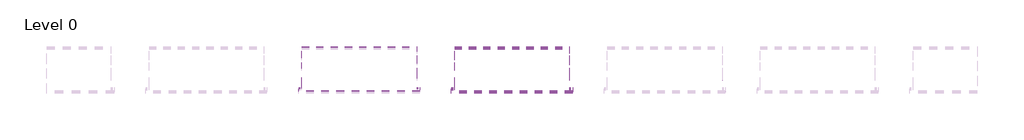
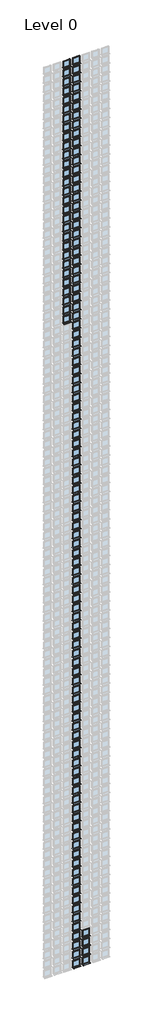
# One storey, part 12 of 75: 133 windows.
"""IFC4 building model written with IfcOpenShell, lengths in millimetres."""

import ifcopenshell
import ifcopenshell.guid

model = None  # the IFC model being written
_history = None  # IfcOwnerHistory: only IFC2X3 demands one
_inside = {}  # id of a spatial element -> (the spatial element, [elements in it])
_under = {}  # id of a project, library or spatial element -> (it, [spatial elements below it])
_declared = {}  # id of a project -> (the project, [libraries it declares])
_typed = {}  # id of a type object -> (the type object, [elements of that type])
_made_of = {}  # id of a material, layer set ... -> (it, [elements and type objects made of it])


def new_model(schema):
    """Start an empty IFC model of exactly this schema.

    Asked for "IFC4X3", IfcOpenShell would pick the latest addendum, in which some entities
    have other attributes; the version numbers below select the first issue.
    IFC2X3 requires an IfcOwnerHistory on every rooted entity: one is made here for all.
    """
    global model, _history
    if schema == "IFC4X3":
        model = ifcopenshell.file(schema_version=(4, 3, 0, 0))
    else:
        model = ifcopenshell.file(schema=schema)
    _inside.clear()
    _under.clear()
    _declared.clear()
    _typed.clear()
    _made_of.clear()
    _history = None
    if model.schema == "IFC2X3":
        org = make("IfcOrganization", Name="unknown")
        user = make(
            "IfcPersonAndOrganization",
            ThePerson=make("IfcPerson", FamilyName="unknown"),
            TheOrganization=org,
        )
        app = make(
            "IfcApplication",
            ApplicationDeveloper=org,
            Version="unknown",
            ApplicationFullName="unknown",
            ApplicationIdentifier="unknown",
        )
        _history = make(
            "IfcOwnerHistory",
            OwningUser=user,
            OwningApplication=app,
            ChangeAction="ADDED",
            CreationDate=0,
        )
    return model


def make(cls, **values):
    """One entity of the class cls with the attributes given. An attribute that is None is left unset."""
    return model.create_entity(
        cls, **{name: value for name, value in values.items() if value is not None}
    )


def rooted(cls, **values):
    """An entity with a GlobalId (a new one), such as an element, a storey or a relation."""
    return make(cls, GlobalId=ifcopenshell.guid.new(), OwnerHistory=_history, **values)


def si_unit(unit_type, name, prefix=None):
    """IfcSIUnit, for example si_unit("LENGTHUNIT", "METRE", prefix="MILLI")."""
    return make("IfcSIUnit", UnitType=unit_type, Prefix=prefix, Name=name)


def assignment(units):
    """IfcUnitAssignment: the units of a project."""
    return None if units is None else make("IfcUnitAssignment", Units=units)


def point(xyz):
    """IfcCartesianPoint."""
    return None if xyz is None else make("IfcCartesianPoint", Coordinates=xyz)


def direction(xyz):
    """IfcDirection."""
    return None if xyz is None else make("IfcDirection", DirectionRatios=xyz)


def frame(location, z_axis=None, x_axis=None):
    """IfcAxis2Placement3D, a coordinate frame: its origin and axes. An axis left out is left unset."""
    return make(
        "IfcAxis2Placement3D",
        Location=point(location),
        Axis=direction(z_axis),
        RefDirection=direction(x_axis),
    )


def origin():
    """The frame at (0, 0, 0) with its axes left unset."""
    return frame((0.0, 0.0, 0.0))


def place(relative_to, where):
    """IfcLocalPlacement: puts the frame where relative to a parent placement (None: the world)."""
    return make(
        "IfcLocalPlacement", PlacementRelTo=relative_to, RelativePlacement=where
    )


def context(
    kind, dimensions, precision=None, world=None, true_north=None, identifier=None
):
    """IfcGeometricRepresentationContext, for example the 3D "Model" context."""
    return make(
        "IfcGeometricRepresentationContext",
        ContextIdentifier=identifier,
        ContextType=kind,
        CoordinateSpaceDimension=dimensions,
        Precision=precision,
        WorldCoordinateSystem=world,
        TrueNorth=true_north,
    )


def project(units=None, contexts=None):
    """IfcProject with its units and contexts."""
    return rooted(
        "IfcProject",
        Name="project",
        RepresentationContexts=contexts,
        UnitsInContext=assignment(units),
    )


def spatial(cls, under=None, at=None, **own):
    """A site, building, storey or space (cls), placed at a placement, below another one or the project."""
    s = rooted(cls, ObjectPlacement=at, **own)
    if under is not None:
        _under.setdefault(under.id(), (under, []))[1].append(s)
    return s


def polyline(points):
    """IfcPolyline through the points."""
    return make("IfcPolyline", Points=[point(p) for p in points])


def outline(outer, holes=None, kind="AREA"):
    """IfcArbitraryClosedProfileDef: a profile drawn as a closed curve; with holes, ...WithVoids."""
    if holes is None:
        return make("IfcArbitraryClosedProfileDef", ProfileType=kind, OuterCurve=outer)
    return make(
        "IfcArbitraryProfileDefWithVoids",
        ProfileType=kind,
        OuterCurve=outer,
        InnerCurves=holes,
    )


def extrude(swept, where, along, depth):
    """IfcExtrudedAreaSolid: the profile swept, set in the frame where, extruded along a direction by depth."""
    return make(
        "IfcExtrudedAreaSolid",
        SweptArea=swept,
        Position=where,
        ExtrudedDirection=direction(along),
        Depth=depth,
    )


def faces_of(points, faces, orient=None, outer=None):
    """IfcFace entities. A face is a list of loops; a loop is a list of indices into points, from 0.

    orient and outer hold one flag for each loop. By default every Orientation is true, the
    first loop of a face is its IfcFaceOuterBound and the others are IfcFaceBound.
    """
    made = []
    for i, loops in enumerate(faces):
        bounds = []
        for j, loop in enumerate(loops):
            is_outer = j == 0 if outer is None else outer[i][j]
            bounds.append(
                make(
                    "IfcFaceOuterBound" if is_outer else "IfcFaceBound",
                    Bound=make("IfcPolyLoop", Polygon=[points[k] for k in loop]),
                    Orientation=True if orient is None else orient[i][j],
                )
            )
        made.append(make("IfcFace", Bounds=bounds))
    return made


def faceted_brep(points, faces, orient=None, outer=None, voids=None):
    """IfcFacetedBrep: a solid bounded by flat faces; with voids (closed shells), ...WithVoids."""
    shared = [point(p) for p in points]
    hull = make("IfcClosedShell", CfsFaces=faces_of(shared, faces, orient, outer))
    if voids is None:
        return make("IfcFacetedBrep", Outer=hull)
    return make(
        "IfcFacetedBrepWithVoids",
        Outer=hull,
        Voids=[
            make(cls, CfsFaces=faces_of(shared, fs, o, b)) for cls, fs, o, b in voids
        ],
    )


def shape(context_of_items, identifier, shape_type, items):
    """IfcShapeRepresentation: the items that make up one representation, for example the "Body"."""
    return make(
        "IfcShapeRepresentation",
        ContextOfItems=context_of_items,
        RepresentationIdentifier=identifier,
        RepresentationType=shape_type,
        Items=items,
    )


def source(mapping_origin, context_of_items, identifier, shape_type, items):
    """IfcRepresentationMap: a shape defined once, which mapped items show again and again."""
    return make(
        "IfcRepresentationMap",
        MappingOrigin=mapping_origin,
        MappedRepresentation=shape(context_of_items, identifier, shape_type, items),
    )


def transform(
    local_origin,
    x_axis=None,
    y_axis=None,
    z_axis=None,
    scale=None,
    scale2=None,
    scale3=None,
    uniform=True,
):
    """IfcCartesianTransformationOperator3D, or its non-uniform kind. x_axis, y_axis, z_axis: its Axis1, 2, 3."""
    if uniform:
        return make(
            "IfcCartesianTransformationOperator3D",
            Axis1=direction(x_axis),
            Axis2=direction(y_axis),
            LocalOrigin=point(local_origin),
            Scale=scale,
            Axis3=direction(z_axis),
        )
    return make(
        "IfcCartesianTransformationOperator3DnonUniform",
        Axis1=direction(x_axis),
        Axis2=direction(y_axis),
        LocalOrigin=point(local_origin),
        Scale=scale,
        Axis3=direction(z_axis),
        Scale2=scale2,
        Scale3=scale3,
    )


def mapped(mapping_source, mapping_target):
    """IfcMappedItem: shows the shape of a source again, moved by a transform."""
    return make(
        "IfcMappedItem", MappingSource=mapping_source, MappingTarget=mapping_target
    )


def made_of(thing, what):
    """Note that an element or type object is made of a material, layer set ...; save() writes the relation."""
    if what is not None:
        _made_of.setdefault(what.id(), (what, []))[1].append(thing)
    return thing


def element(
    cls,
    number,
    at=None,
    inside=None,
    cuts=None,
    type_object=None,
    material=None,
    context=None,
    identifier="Body",
    shape_type=None,
    held_by="IfcProductDefinitionShape",
    body=None,
    shapes=None,
    **own,
):
    """One element of the class cls, such as IfcWall. Its Tag is "e" and its number.

    at: its placement. inside: the storey or other place that contains it. cuts: it is an
    opening in that element (IfcRelVoidsElement). A single representation is given by context,
    identifier, shape_type and body (its items); several are given by shapes. held_by: the class
    of the entity that holds the representations. save() writes the other relations.
    """
    e = rooted(cls, Tag="e%d" % number, ObjectPlacement=at, **own)
    if body is not None:
        shapes = [shape(context, identifier, shape_type, body)]
    if shapes is not None:
        e.Representation = make(held_by, Representations=shapes)
    if inside is not None:
        _inside.setdefault(inside.id(), (inside, []))[1].append(e)
    if cuts is not None:
        rooted(
            "IfcRelVoidsElement", RelatingBuildingElement=cuts, RelatedOpeningElement=e
        )
    if type_object is not None:
        _typed.setdefault(type_object.id(), (type_object, []))[1].append(e)
    return made_of(e, material)


def aggregate(whole, parts):
    """IfcRelAggregates: a whole, such as a stair, and the parts it consists of."""
    return rooted("IfcRelAggregates", RelatingObject=whole, RelatedObjects=parts)


def save(model, path):
    """Write the relations noted so far, then the file.

    IfcRelAggregates (storeys below a building ...), IfcRelContainedInSpatialStructure (elements
    in a storey), IfcRelDefinesByType, IfcRelAssociatesMaterial and IfcRelDeclares: one each for
    every whole, place, type object, material and project.
    """
    for whole, parts in _under.values():
        aggregate(whole, parts)
    for where, things in _inside.values():
        rooted(
            "IfcRelContainedInSpatialStructure",
            RelatedElements=things,
            RelatingStructure=where,
        )
    for kind, things in _typed.values():
        rooted("IfcRelDefinesByType", RelatedObjects=things, RelatingType=kind)
    for what, things in _made_of.values():
        rooted("IfcRelAssociatesMaterial", RelatedObjects=things, RelatingMaterial=what)
    for by, libraries in _declared.values():
        rooted("IfcRelDeclares", RelatingContext=by, RelatedDefinitions=libraries)
    model.write(path)


def windows_sgl_plain_square_green_b9caa461(model_context):
    return source(origin(), model_context, "Body", "SolidModel", [
        extrude(outline(polyline([(-480.0, -161.5434322), (-480.0, -136.5434322), (-455.0, -136.5434322), (-455.0, 20.4565678), (455.0, 20.4565678), (455.0, -136.5434322), (480.0, -136.5434322), (480.0, -161.5434322), (-480.0, -161.5434322)])), frame((0.0, 0.0, 1200.0), z_axis=(0.0, 0.0, 1.0), x_axis=(1.0, 0.0, 0.0)), (0.0, 0.0, 1.0), 25.0),
        faceted_brep([(-455.0, 20.4565678, 1200.0), (455.0, 20.4565678, 1200.0), (455.0, 20.4565678, 2110.0), (-455.0, 20.4565678, 2110.0), (-395.0, 20.4565678, 2050.0), (395.0, 20.4565678, 2050.0), (395.0, 20.4565678, 1275.0), (-395.0, 20.4565678, 1275.0), (-455.0, 103.4565678, 2110.0), (-455.0, 103.4565678, 1251.0), (-455.0, 118.4565678, 1249.68767), (-455.0, 118.4565678, 1244.7449676), (-455.0, 190.9565678, 1233.8088847), (-455.0, 190.9565678, 1200.0), (455.0, 103.4565678, 2110.0), (455.0, 103.4565678, 1251.0), (-415.0, 103.4565678, 2070.0), (-415.0, 103.4565678, 1263.0), (415.0, 103.4565678, 1263.0), (415.0, 103.4565678, 2070.0), (-415.0, 38.4565678, 2070.0), (-415.0, 38.4565678, 1263.0), (415.0, 38.4565678, 2070.0), (415.0, 38.4565678, 1263.0), (-395.0, 38.4565678, 2050.0), (-395.0, 38.4565678, 1275.0), (395.0, 38.4565678, 1275.0), (395.0, 38.4565678, 2050.0), (455.0, 190.9565678, 1200.0), (455.0, 190.9565678, 1233.8088847), (455.0, 118.4565678, 1244.7449676), (455.0, 118.4565678, 1249.68767)], [[[0, 1, 2, 3], [4, 5, 6, 7]], [[0, 3, 8, 9, 10, 11, 12, 13]], [[9, 8, 14, 15], [16, 17, 18, 19]], [[17, 16, 20, 21]], [[20, 22, 23, 21], [24, 25, 26, 27]], [[24, 4, 7, 25]], [[3, 2, 14, 8]], [[16, 19, 22, 20]], [[5, 4, 24, 27]], [[15, 14, 2, 1, 28, 29, 30, 31]], [[19, 18, 23, 22]], [[5, 27, 26, 6]], [[28, 1, 0, 13]], [[29, 28, 13, 12]], [[30, 29, 12, 11]], [[31, 30, 11, 10]], [[15, 31, 10, 9]], [[21, 23, 18, 17]], [[7, 6, 26, 25]]]),
        extrude(outline(polyline([(385.0, 67.4565678), (-385.0, 67.4565678), (-385.0, 91.4565678), (385.0, 91.4565678), (385.0, 67.4565678)])), frame((0.0, 0.0, 1293.0), z_axis=(0.0, 0.0, 1.0), x_axis=(1.0, 0.0, 0.0)), (0.0, 0.0, 1.0), 747.0),
        faceted_brep([(-425.0, 103.4565678, 2080.0), (-425.0, 109.2300705, 2080.0), (-425.0, 109.2300705, 1253.0), (-425.0, 103.4565678, 1253.0), (-415.0, 38.4565678, 2070.0), (-415.0, 103.4565678, 2070.0), (-415.0, 103.4565678, 1263.0), (-415.0, 38.4565678, 1263.0), (-375.0, 52.9494677, 2030.0), (-385.1480377, 38.4565678, 2040.1480377), (-385.1480377, 38.4565678, 1292.8519623), (-375.0, 52.9494677, 1303.0), (-375.0, 67.4565678, 2030.0), (-375.0, 67.4565678, 1303.0), (-385.0, 91.4565678, 2040.0), (-385.0, 67.4565678, 2040.0), (-385.0, 67.4565678, 1293.0), (-385.0, 91.4565678, 1293.0), (-375.0, 109.2300705, 2030.0), (-375.0, 91.4565678, 2030.0), (-375.0, 91.4565678, 1303.0), (-375.0, 109.2300705, 1303.0), (-392.4457548, 115.0035732, 2047.4457548), (-392.4457548, 115.0035732, 1285.5542452), (-414.2153903, 115.0035732, 2069.2153903), (-414.2153903, 115.0035732, 1263.7846097), (425.0, 109.2300705, 1253.0), (425.0, 103.4565678, 1253.0), (415.0, 103.4565678, 1263.0), (415.0, 38.4565678, 1263.0), (385.1480377, 38.4565678, 1292.8519623), (375.0, 52.9494677, 1303.0), (375.0, 67.4565678, 1303.0), (385.0, 67.4565678, 1293.0), (385.0, 91.4565678, 1293.0), (375.0, 91.4565678, 1303.0), (375.0, 109.2300705, 1303.0), (392.4457548, 115.0035732, 1285.5542452), (414.2153903, 115.0035732, 1263.7846097), (425.0, 109.2300705, 2080.0), (425.0, 103.4565678, 2080.0), (415.0, 103.4565678, 2070.0), (415.0, 38.4565678, 2070.0), (385.1480377, 38.4565678, 2040.1480377), (375.0, 52.9494677, 2030.0), (375.0, 67.4565678, 2030.0), (385.0, 67.4565678, 2040.0), (385.0, 91.4565678, 2040.0), (375.0, 91.4565678, 2030.0), (375.0, 109.2300705, 2030.0), (392.4457548, 115.0035732, 2047.4457548), (414.2153903, 115.0035732, 2069.2153903)], [[[0, 1, 2, 3]], [[4, 5, 6, 7]], [[8, 9, 10, 11]], [[12, 8, 11, 13]], [[14, 15, 16, 17]], [[18, 19, 20, 21]], [[22, 18, 21, 23]], [[1, 24, 25, 2]], [[3, 2, 26, 27]], [[7, 6, 28, 29]], [[11, 10, 30, 31]], [[13, 11, 31, 32]], [[17, 16, 33, 34]], [[21, 20, 35, 36]], [[23, 21, 36, 37]], [[2, 25, 38, 26]], [[27, 26, 39, 40]], [[29, 28, 41, 42]], [[31, 30, 43, 44]], [[32, 31, 44, 45]], [[34, 33, 46, 47]], [[36, 35, 48, 49]], [[37, 36, 49, 50]], [[26, 38, 51, 39]], [[40, 39, 1, 0]], [[3, 27, 40, 0], [5, 41, 28, 6]], [[42, 41, 5, 4]], [[7, 29, 42, 4], [9, 43, 30, 10]], [[44, 43, 9, 8]], [[45, 44, 8, 12]], [[15, 46, 33, 16], [13, 32, 45, 12]], [[47, 46, 15, 14]], [[17, 34, 47, 14], [19, 48, 35, 20]], [[49, 48, 19, 18]], [[50, 49, 18, 22]], [[24, 51, 38, 25], [23, 37, 50, 22]], [[39, 51, 24, 1]]]),
    ])


model = new_model("IFC4")

# Units and contexts
model_context = context("Model", 3, world=origin())
ifc_project = project(units=[si_unit("LENGTHUNIT", "METRE", prefix="MILLI")], contexts=[model_context])

# Site, building, storey
site = spatial("IfcSite", under=ifc_project)
building = spatial("IfcBuilding", under=site)
storey = spatial("IfcBuildingStorey", under=building, Name="Level 0", Elevation=0.0)

# Windows
placement = place(None, origin())
windows_sgl_plain_square_green_shape = windows_sgl_plain_square_green_b9caa461(model_context)
element("IfcWindow", 1, ObjectType="Windows_Sgl_Plain : Square Green", at=placement, inside=storey, context=model_context, shape_type="MappedRepresentation", body=[
    mapped(windows_sgl_plain_square_green_shape, transform((-36933.7647367, 3061.0736592, 41224.2424242), x_axis=(1.0, 0.0, 0.0), y_axis=(0.0, 1.0, 0.0), z_axis=(0.0, 0.0, 1.0))),
])
element("IfcWindow", 2, ObjectType="Windows_Sgl_Plain : Square Green", at=placement, inside=storey, context=model_context, shape_type="MappedRepresentation", body=[
    mapped(windows_sgl_plain_square_green_shape, transform((-38145.8859488, 3061.0736592, 113951.5151515), x_axis=(1.0, 0.0, 0.0), y_axis=(0.0, 1.0, 0.0), z_axis=(0.0, 0.0, 1.0))),
])
element("IfcWindow", 3, ObjectType="Windows_Sgl_Plain : Square Green", at=placement, inside=storey, context=model_context, shape_type="MappedRepresentation", body=[
    mapped(windows_sgl_plain_square_green_shape, transform((-38145.8859488, 3061.0736592, 115163.6363636), x_axis=(1.0, 0.0, 0.0), y_axis=(0.0, 1.0, 0.0), z_axis=(0.0, 0.0, 1.0))),
])
element("IfcWindow", 4, ObjectType="Windows_Sgl_Plain : Square Normal", at=placement, inside=storey, context=model_context, shape_type="MappedRepresentation", body=[
    mapped(windows_sgl_plain_square_green_shape, transform((-38145.8859488, 3061.0736592, 41224.2424242), x_axis=(1.0, 0.0, 0.0), y_axis=(0.0, 1.0, 0.0), z_axis=(0.0, 0.0, 1.0))),
])
element("IfcWindow", 5, ObjectType="Windows_Sgl_Plain : Square Normal", at=placement, inside=storey, context=model_context, shape_type="MappedRepresentation", body=[
    mapped(windows_sgl_plain_square_green_shape, transform((-38145.8859488, 3061.0736592, 42436.3636364), x_axis=(1.0, 0.0, 0.0), y_axis=(0.0, 1.0, 0.0), z_axis=(0.0, 0.0, 1.0))),
])
element("IfcWindow", 6, ObjectType="Windows_Sgl_Plain : Square Normal", at=placement, inside=storey, context=model_context, shape_type="MappedRepresentation", body=[
    mapped(windows_sgl_plain_square_green_shape, transform((-36933.7647367, 3061.0736592, 42436.3636364), x_axis=(1.0, 0.0, 0.0), y_axis=(0.0, 1.0, 0.0), z_axis=(0.0, 0.0, 1.0))),
])
element("IfcWindow", 7, ObjectType="Windows_Sgl_Plain : Square Normal", at=placement, inside=storey, context=model_context, shape_type="MappedRepresentation", body=[
    mapped(windows_sgl_plain_square_green_shape, transform((-38145.8859488, 3061.0736592, 43648.4848485), x_axis=(1.0, 0.0, 0.0), y_axis=(0.0, 1.0, 0.0), z_axis=(0.0, 0.0, 1.0))),
])
element("IfcWindow", 8, ObjectType="Windows_Sgl_Plain : Square Normal", at=placement, inside=storey, context=model_context, shape_type="MappedRepresentation", body=[
    mapped(windows_sgl_plain_square_green_shape, transform((-38145.8859488, 3061.0736592, 44860.6060606), x_axis=(1.0, 0.0, 0.0), y_axis=(0.0, 1.0, 0.0), z_axis=(0.0, 0.0, 1.0))),
])
element("IfcWindow", 9, ObjectType="Windows_Sgl_Plain : Square Normal", at=placement, inside=storey, context=model_context, shape_type="MappedRepresentation", body=[
    mapped(windows_sgl_plain_square_green_shape, transform((-38145.8859488, 3061.0736592, 46072.7272727), x_axis=(1.0, 0.0, 0.0), y_axis=(0.0, 1.0, 0.0), z_axis=(0.0, 0.0, 1.0))),
])
element("IfcWindow", 10, ObjectType="Windows_Sgl_Plain : Square Normal", at=placement, inside=storey, context=model_context, shape_type="MappedRepresentation", body=[
    mapped(windows_sgl_plain_square_green_shape, transform((-38145.8859488, 3061.0736592, 47284.8484848), x_axis=(1.0, 0.0, 0.0), y_axis=(0.0, 1.0, 0.0), z_axis=(0.0, 0.0, 1.0))),
])
element("IfcWindow", 11, ObjectType="Windows_Sgl_Plain : Square Normal", at=placement, inside=storey, context=model_context, shape_type="MappedRepresentation", body=[
    mapped(windows_sgl_plain_square_green_shape, transform((-38145.8859488, 3061.0736592, 48496.969697), x_axis=(1.0, 0.0, 0.0), y_axis=(0.0, 1.0, 0.0), z_axis=(0.0, 0.0, 1.0))),
])
element("IfcWindow", 12, ObjectType="Windows_Sgl_Plain : Square Normal", at=placement, inside=storey, context=model_context, shape_type="MappedRepresentation", body=[
    mapped(windows_sgl_plain_square_green_shape, transform((-38145.8859488, 3061.0736592, 49709.0909091), x_axis=(1.0, 0.0, 0.0), y_axis=(0.0, 1.0, 0.0), z_axis=(0.0, 0.0, 1.0))),
])
element("IfcWindow", 13, ObjectType="Windows_Sgl_Plain : Square Normal", at=placement, inside=storey, context=model_context, shape_type="MappedRepresentation", body=[
    mapped(windows_sgl_plain_square_green_shape, transform((-38145.8859488, 3061.0736592, 50921.2121212), x_axis=(1.0, 0.0, 0.0), y_axis=(0.0, 1.0, 0.0), z_axis=(0.0, 0.0, 1.0))),
])
element("IfcWindow", 14, ObjectType="Windows_Sgl_Plain : Square Normal", at=placement, inside=storey, context=model_context, shape_type="MappedRepresentation", body=[
    mapped(windows_sgl_plain_square_green_shape, transform((-38145.8859488, 3061.0736592, 52133.3333333), x_axis=(1.0, 0.0, 0.0), y_axis=(0.0, 1.0, 0.0), z_axis=(0.0, 0.0, 1.0))),
])
element("IfcWindow", 15, ObjectType="Windows_Sgl_Plain : Square Normal", at=placement, inside=storey, context=model_context, shape_type="MappedRepresentation", body=[
    mapped(windows_sgl_plain_square_green_shape, transform((-38145.8859488, 3061.0736592, 53345.4545455), x_axis=(1.0, 0.0, 0.0), y_axis=(0.0, 1.0, 0.0), z_axis=(0.0, 0.0, 1.0))),
])
element("IfcWindow", 16, ObjectType="Windows_Sgl_Plain : Square Normal", at=placement, inside=storey, context=model_context, shape_type="MappedRepresentation", body=[
    mapped(windows_sgl_plain_square_green_shape, transform((-38145.8859488, 3061.0736592, 54557.5757576), x_axis=(1.0, 0.0, 0.0), y_axis=(0.0, 1.0, 0.0), z_axis=(0.0, 0.0, 1.0))),
])
element("IfcWindow", 17, ObjectType="Windows_Sgl_Plain : Square Normal", at=placement, inside=storey, context=model_context, shape_type="MappedRepresentation", body=[
    mapped(windows_sgl_plain_square_green_shape, transform((-38145.8859488, 3061.0736592, 55769.6969697), x_axis=(1.0, 0.0, 0.0), y_axis=(0.0, 1.0, 0.0), z_axis=(0.0, 0.0, 1.0))),
])
element("IfcWindow", 18, ObjectType="Windows_Sgl_Plain : Square Normal", at=placement, inside=storey, context=model_context, shape_type="MappedRepresentation", body=[
    mapped(windows_sgl_plain_square_green_shape, transform((-38145.8859488, 3061.0736592, 56981.8181818), x_axis=(1.0, 0.0, 0.0), y_axis=(0.0, 1.0, 0.0), z_axis=(0.0, 0.0, 1.0))),
])
element("IfcWindow", 19, ObjectType="Windows_Sgl_Plain : Square Normal", at=placement, inside=storey, context=model_context, shape_type="MappedRepresentation", body=[
    mapped(windows_sgl_plain_square_green_shape, transform((-38145.8859488, 3061.0736592, 58193.9393939), x_axis=(1.0, 0.0, 0.0), y_axis=(0.0, 1.0, 0.0), z_axis=(0.0, 0.0, 1.0))),
])
element("IfcWindow", 20, ObjectType="Windows_Sgl_Plain : Square Normal", at=placement, inside=storey, context=model_context, shape_type="MappedRepresentation", body=[
    mapped(windows_sgl_plain_square_green_shape, transform((-38145.8859488, 3061.0736592, 59406.0606061), x_axis=(1.0, 0.0, 0.0), y_axis=(0.0, 1.0, 0.0), z_axis=(0.0, 0.0, 1.0))),
])
element("IfcWindow", 21, ObjectType="Windows_Sgl_Plain : Square Normal", at=placement, inside=storey, context=model_context, shape_type="MappedRepresentation", body=[
    mapped(windows_sgl_plain_square_green_shape, transform((-38145.8859488, 3061.0736592, 60618.1818182), x_axis=(1.0, 0.0, 0.0), y_axis=(0.0, 1.0, 0.0), z_axis=(0.0, 0.0, 1.0))),
])
element("IfcWindow", 22, ObjectType="Windows_Sgl_Plain : Square Normal", at=placement, inside=storey, context=model_context, shape_type="MappedRepresentation", body=[
    mapped(windows_sgl_plain_square_green_shape, transform((-38145.8859488, 3061.0736592, 61830.3030303), x_axis=(1.0, 0.0, 0.0), y_axis=(0.0, 1.0, 0.0), z_axis=(0.0, 0.0, 1.0))),
])
element("IfcWindow", 23, ObjectType="Windows_Sgl_Plain : Square Normal", at=placement, inside=storey, context=model_context, shape_type="MappedRepresentation", body=[
    mapped(windows_sgl_plain_square_green_shape, transform((-38145.8859488, 3061.0736592, 63042.4242424), x_axis=(1.0, 0.0, 0.0), y_axis=(0.0, 1.0, 0.0), z_axis=(0.0, 0.0, 1.0))),
])
element("IfcWindow", 24, ObjectType="Windows_Sgl_Plain : Square Normal", at=placement, inside=storey, context=model_context, shape_type="MappedRepresentation", body=[
    mapped(windows_sgl_plain_square_green_shape, transform((-38145.8859488, 3061.0736592, 64254.5454545), x_axis=(1.0, 0.0, 0.0), y_axis=(0.0, 1.0, 0.0), z_axis=(0.0, 0.0, 1.0))),
])
element("IfcWindow", 25, ObjectType="Windows_Sgl_Plain : Square Normal", at=placement, inside=storey, context=model_context, shape_type="MappedRepresentation", body=[
    mapped(windows_sgl_plain_square_green_shape, transform((-38145.8859488, 3061.0736592, 65466.6666667), x_axis=(1.0, 0.0, 0.0), y_axis=(0.0, 1.0, 0.0), z_axis=(0.0, 0.0, 1.0))),
])
element("IfcWindow", 26, ObjectType="Windows_Sgl_Plain : Square Normal", at=placement, inside=storey, context=model_context, shape_type="MappedRepresentation", body=[
    mapped(windows_sgl_plain_square_green_shape, transform((-38145.8859488, 3061.0736592, 66678.7878788), x_axis=(1.0, 0.0, 0.0), y_axis=(0.0, 1.0, 0.0), z_axis=(0.0, 0.0, 1.0))),
])
element("IfcWindow", 27, ObjectType="Windows_Sgl_Plain : Square Normal", at=placement, inside=storey, context=model_context, shape_type="MappedRepresentation", body=[
    mapped(windows_sgl_plain_square_green_shape, transform((-38145.8859488, 3061.0736592, 67890.9090909), x_axis=(1.0, 0.0, 0.0), y_axis=(0.0, 1.0, 0.0), z_axis=(0.0, 0.0, 1.0))),
])
element("IfcWindow", 28, ObjectType="Windows_Sgl_Plain : Square Normal", at=placement, inside=storey, context=model_context, shape_type="MappedRepresentation", body=[
    mapped(windows_sgl_plain_square_green_shape, transform((-38145.8859488, 3061.0736592, 69103.030303), x_axis=(1.0, 0.0, 0.0), y_axis=(0.0, 1.0, 0.0), z_axis=(0.0, 0.0, 1.0))),
])
element("IfcWindow", 29, ObjectType="Windows_Sgl_Plain : Square Normal", at=placement, inside=storey, context=model_context, shape_type="MappedRepresentation", body=[
    mapped(windows_sgl_plain_square_green_shape, transform((-38145.8859488, 3061.0736592, 70315.1515152), x_axis=(1.0, 0.0, 0.0), y_axis=(0.0, 1.0, 0.0), z_axis=(0.0, 0.0, 1.0))),
])
element("IfcWindow", 30, ObjectType="Windows_Sgl_Plain : Square Normal", at=placement, inside=storey, context=model_context, shape_type="MappedRepresentation", body=[
    mapped(windows_sgl_plain_square_green_shape, transform((-38145.8859488, 3061.0736592, 71527.2727273), x_axis=(1.0, 0.0, 0.0), y_axis=(0.0, 1.0, 0.0), z_axis=(0.0, 0.0, 1.0))),
])
element("IfcWindow", 31, ObjectType="Windows_Sgl_Plain : Square Normal", at=placement, inside=storey, context=model_context, shape_type="MappedRepresentation", body=[
    mapped(windows_sgl_plain_square_green_shape, transform((-38145.8859488, 3061.0736592, 72739.3939394), x_axis=(1.0, 0.0, 0.0), y_axis=(0.0, 1.0, 0.0), z_axis=(0.0, 0.0, 1.0))),
])
element("IfcWindow", 32, ObjectType="Windows_Sgl_Plain : Square Normal", at=placement, inside=storey, context=model_context, shape_type="MappedRepresentation", body=[
    mapped(windows_sgl_plain_square_green_shape, transform((-38145.8859488, 3061.0736592, 73951.5151515), x_axis=(1.0, 0.0, 0.0), y_axis=(0.0, 1.0, 0.0), z_axis=(0.0, 0.0, 1.0))),
])
element("IfcWindow", 33, ObjectType="Windows_Sgl_Plain : Square Normal", at=placement, inside=storey, context=model_context, shape_type="MappedRepresentation", body=[
    mapped(windows_sgl_plain_square_green_shape, transform((-38145.8859488, 3061.0736592, 75163.6363636), x_axis=(1.0, 0.0, 0.0), y_axis=(0.0, 1.0, 0.0), z_axis=(0.0, 0.0, 1.0))),
])
element("IfcWindow", 34, ObjectType="Windows_Sgl_Plain : Square Normal", at=placement, inside=storey, context=model_context, shape_type="MappedRepresentation", body=[
    mapped(windows_sgl_plain_square_green_shape, transform((-38145.8859488, 3061.0736592, 76375.7575758), x_axis=(1.0, 0.0, 0.0), y_axis=(0.0, 1.0, 0.0), z_axis=(0.0, 0.0, 1.0))),
])
element("IfcWindow", 35, ObjectType="Windows_Sgl_Plain : Square Normal", at=placement, inside=storey, context=model_context, shape_type="MappedRepresentation", body=[
    mapped(windows_sgl_plain_square_green_shape, transform((-38145.8859488, 3061.0736592, 77587.8787879), x_axis=(1.0, 0.0, 0.0), y_axis=(0.0, 1.0, 0.0), z_axis=(0.0, 0.0, 1.0))),
])
element("IfcWindow", 36, ObjectType="Windows_Sgl_Plain : Square Normal", at=placement, inside=storey, context=model_context, shape_type="MappedRepresentation", body=[
    mapped(windows_sgl_plain_square_green_shape, transform((-38145.8859488, 3061.0736592, 78800.0), x_axis=(1.0, 0.0, 0.0), y_axis=(0.0, 1.0, 0.0), z_axis=(0.0, 0.0, 1.0))),
])
element("IfcWindow", 37, ObjectType="Windows_Sgl_Plain : Square Normal", at=placement, inside=storey, context=model_context, shape_type="MappedRepresentation", body=[
    mapped(windows_sgl_plain_square_green_shape, transform((-38145.8859488, 3061.0736592, 80012.1212121), x_axis=(1.0, 0.0, 0.0), y_axis=(0.0, 1.0, 0.0), z_axis=(0.0, 0.0, 1.0))),
])
element("IfcWindow", 38, ObjectType="Windows_Sgl_Plain : Square Normal", at=placement, inside=storey, context=model_context, shape_type="MappedRepresentation", body=[
    mapped(windows_sgl_plain_square_green_shape, transform((-38145.8859488, 3061.0736592, 81224.2424242), x_axis=(1.0, 0.0, 0.0), y_axis=(0.0, 1.0, 0.0), z_axis=(0.0, 0.0, 1.0))),
])
element("IfcWindow", 39, ObjectType="Windows_Sgl_Plain : Square Normal", at=placement, inside=storey, context=model_context, shape_type="MappedRepresentation", body=[
    mapped(windows_sgl_plain_square_green_shape, transform((-38145.8859488, 3061.0736592, 82436.3636364), x_axis=(1.0, 0.0, 0.0), y_axis=(0.0, 1.0, 0.0), z_axis=(0.0, 0.0, 1.0))),
])
element("IfcWindow", 40, ObjectType="Windows_Sgl_Plain : Square Normal", at=placement, inside=storey, context=model_context, shape_type="MappedRepresentation", body=[
    mapped(windows_sgl_plain_square_green_shape, transform((-38145.8859488, 3061.0736592, 83648.4848485), x_axis=(1.0, 0.0, 0.0), y_axis=(0.0, 1.0, 0.0), z_axis=(0.0, 0.0, 1.0))),
])
element("IfcWindow", 41, ObjectType="Windows_Sgl_Plain : Square Normal", at=placement, inside=storey, context=model_context, shape_type="MappedRepresentation", body=[
    mapped(windows_sgl_plain_square_green_shape, transform((-38145.8859488, 3061.0736592, 84860.6060606), x_axis=(1.0, 0.0, 0.0), y_axis=(0.0, 1.0, 0.0), z_axis=(0.0, 0.0, 1.0))),
])
element("IfcWindow", 42, ObjectType="Windows_Sgl_Plain : Square Normal", at=placement, inside=storey, context=model_context, shape_type="MappedRepresentation", body=[
    mapped(windows_sgl_plain_square_green_shape, transform((-38145.8859488, 3061.0736592, 86072.7272727), x_axis=(1.0, 0.0, 0.0), y_axis=(0.0, 1.0, 0.0), z_axis=(0.0, 0.0, 1.0))),
])
element("IfcWindow", 43, ObjectType="Windows_Sgl_Plain : Square Normal", at=placement, inside=storey, context=model_context, shape_type="MappedRepresentation", body=[
    mapped(windows_sgl_plain_square_green_shape, transform((-38145.8859488, 3061.0736592, 87284.8484848), x_axis=(1.0, 0.0, 0.0), y_axis=(0.0, 1.0, 0.0), z_axis=(0.0, 0.0, 1.0))),
])
element("IfcWindow", 44, ObjectType="Windows_Sgl_Plain : Square Normal", at=placement, inside=storey, context=model_context, shape_type="MappedRepresentation", body=[
    mapped(windows_sgl_plain_square_green_shape, transform((-38145.8859488, 3061.0736592, 88496.969697), x_axis=(1.0, 0.0, 0.0), y_axis=(0.0, 1.0, 0.0), z_axis=(0.0, 0.0, 1.0))),
])
element("IfcWindow", 45, ObjectType="Windows_Sgl_Plain : Square Normal", at=placement, inside=storey, context=model_context, shape_type="MappedRepresentation", body=[
    mapped(windows_sgl_plain_square_green_shape, transform((-38145.8859488, 3061.0736592, 89709.0909091), x_axis=(1.0, 0.0, 0.0), y_axis=(0.0, 1.0, 0.0), z_axis=(0.0, 0.0, 1.0))),
])
element("IfcWindow", 46, ObjectType="Windows_Sgl_Plain : Square Normal", at=placement, inside=storey, context=model_context, shape_type="MappedRepresentation", body=[
    mapped(windows_sgl_plain_square_green_shape, transform((-38145.8859488, 3061.0736592, 90921.2121212), x_axis=(1.0, 0.0, 0.0), y_axis=(0.0, 1.0, 0.0), z_axis=(0.0, 0.0, 1.0))),
])
element("IfcWindow", 47, ObjectType="Windows_Sgl_Plain : Square Normal", at=placement, inside=storey, context=model_context, shape_type="MappedRepresentation", body=[
    mapped(windows_sgl_plain_square_green_shape, transform((-38145.8859488, 3061.0736592, 96981.8181818), x_axis=(1.0, 0.0, 0.0), y_axis=(0.0, 1.0, 0.0), z_axis=(0.0, 0.0, 1.0))),
])
element("IfcWindow", 48, ObjectType="Windows_Sgl_Plain : Square Normal", at=placement, inside=storey, context=model_context, shape_type="MappedRepresentation", body=[
    mapped(windows_sgl_plain_square_green_shape, transform((-38145.8859488, 3061.0736592, 98193.9393939), x_axis=(1.0, 0.0, 0.0), y_axis=(0.0, 1.0, 0.0), z_axis=(0.0, 0.0, 1.0))),
])
element("IfcWindow", 49, ObjectType="Windows_Sgl_Plain : Square Normal", at=placement, inside=storey, context=model_context, shape_type="MappedRepresentation", body=[
    mapped(windows_sgl_plain_square_green_shape, transform((-38145.8859488, 3061.0736592, 99406.0606061), x_axis=(1.0, 0.0, 0.0), y_axis=(0.0, 1.0, 0.0), z_axis=(0.0, 0.0, 1.0))),
])
element("IfcWindow", 50, ObjectType="Windows_Sgl_Plain : Square Normal", at=placement, inside=storey, context=model_context, shape_type="MappedRepresentation", body=[
    mapped(windows_sgl_plain_square_green_shape, transform((-38145.8859488, 3061.0736592, 100618.1818182), x_axis=(1.0, 0.0, 0.0), y_axis=(0.0, 1.0, 0.0), z_axis=(0.0, 0.0, 1.0))),
])
element("IfcWindow", 51, ObjectType="Windows_Sgl_Plain : Square Normal", at=placement, inside=storey, context=model_context, shape_type="MappedRepresentation", body=[
    mapped(windows_sgl_plain_square_green_shape, transform((-38145.8859488, 3061.0736592, 101830.3030303), x_axis=(1.0, 0.0, 0.0), y_axis=(0.0, 1.0, 0.0), z_axis=(0.0, 0.0, 1.0))),
])
element("IfcWindow", 52, ObjectType="Windows_Sgl_Plain : Square Normal", at=placement, inside=storey, context=model_context, shape_type="MappedRepresentation", body=[
    mapped(windows_sgl_plain_square_green_shape, transform((-38145.8859488, 3061.0736592, 103042.4242424), x_axis=(1.0, 0.0, 0.0), y_axis=(0.0, 1.0, 0.0), z_axis=(0.0, 0.0, 1.0))),
])
element("IfcWindow", 53, ObjectType="Windows_Sgl_Plain : Square Normal", at=placement, inside=storey, context=model_context, shape_type="MappedRepresentation", body=[
    mapped(windows_sgl_plain_square_green_shape, transform((-38145.8859488, 3061.0736592, 104254.5454545), x_axis=(1.0, 0.0, 0.0), y_axis=(0.0, 1.0, 0.0), z_axis=(0.0, 0.0, 1.0))),
])
element("IfcWindow", 54, ObjectType="Windows_Sgl_Plain : Square Normal", at=placement, inside=storey, context=model_context, shape_type="MappedRepresentation", body=[
    mapped(windows_sgl_plain_square_green_shape, transform((-38145.8859488, 3061.0736592, 105466.6666667), x_axis=(1.0, 0.0, 0.0), y_axis=(0.0, 1.0, 0.0), z_axis=(0.0, 0.0, 1.0))),
])
element("IfcWindow", 55, ObjectType="Windows_Sgl_Plain : Square Normal", at=placement, inside=storey, context=model_context, shape_type="MappedRepresentation", body=[
    mapped(windows_sgl_plain_square_green_shape, transform((-38145.8859488, 3061.0736592, 106678.7878788), x_axis=(1.0, 0.0, 0.0), y_axis=(0.0, 1.0, 0.0), z_axis=(0.0, 0.0, 1.0))),
])
element("IfcWindow", 56, ObjectType="Windows_Sgl_Plain : Square Normal", at=placement, inside=storey, context=model_context, shape_type="MappedRepresentation", body=[
    mapped(windows_sgl_plain_square_green_shape, transform((-38145.8859488, 3061.0736592, 107890.9090909), x_axis=(1.0, 0.0, 0.0), y_axis=(0.0, 1.0, 0.0), z_axis=(0.0, 0.0, 1.0))),
])
element("IfcWindow", 57, ObjectType="Windows_Sgl_Plain : Square Normal", at=placement, inside=storey, context=model_context, shape_type="MappedRepresentation", body=[
    mapped(windows_sgl_plain_square_green_shape, transform((-38145.8859488, 3061.0736592, 109103.030303), x_axis=(1.0, 0.0, 0.0), y_axis=(0.0, 1.0, 0.0), z_axis=(0.0, 0.0, 1.0))),
])
element("IfcWindow", 58, ObjectType="Windows_Sgl_Plain : Square Normal", at=placement, inside=storey, context=model_context, shape_type="MappedRepresentation", body=[
    mapped(windows_sgl_plain_square_green_shape, transform((-38145.8859488, 3061.0736592, 110315.1515152), x_axis=(1.0, 0.0, 0.0), y_axis=(0.0, 1.0, 0.0), z_axis=(0.0, 0.0, 1.0))),
])
element("IfcWindow", 59, ObjectType="Windows_Sgl_Plain : Square Normal", at=placement, inside=storey, context=model_context, shape_type="MappedRepresentation", body=[
    mapped(windows_sgl_plain_square_green_shape, transform((-38145.8859488, 3061.0736592, 111527.2727273), x_axis=(1.0, 0.0, 0.0), y_axis=(0.0, 1.0, 0.0), z_axis=(0.0, 0.0, 1.0))),
])
element("IfcWindow", 60, ObjectType="Windows_Sgl_Plain : Square Normal", at=placement, inside=storey, context=model_context, shape_type="MappedRepresentation", body=[
    mapped(windows_sgl_plain_square_green_shape, transform((-38145.8859488, 3061.0736592, 112739.3939394), x_axis=(1.0, 0.0, 0.0), y_axis=(0.0, 1.0, 0.0), z_axis=(0.0, 0.0, 1.0))),
])
element("IfcWindow", 61, ObjectType="Windows_Sgl_Plain : Square Normal", at=placement, inside=storey, context=model_context, shape_type="MappedRepresentation", body=[
    mapped(windows_sgl_plain_square_green_shape, transform((-38145.8859488, 3061.0736592, 116375.7575758), x_axis=(1.0, 0.0, 0.0), y_axis=(0.0, 1.0, 0.0), z_axis=(0.0, 0.0, 1.0))),
])
element("IfcWindow", 62, ObjectType="Windows_Sgl_Plain : Square Normal", at=placement, inside=storey, context=model_context, shape_type="MappedRepresentation", body=[
    mapped(windows_sgl_plain_square_green_shape, transform((-38145.8859488, 3061.0736592, 117587.8787879), x_axis=(1.0, 0.0, 0.0), y_axis=(0.0, 1.0, 0.0), z_axis=(0.0, 0.0, 1.0))),
])
element("IfcWindow", 63, ObjectType="Windows_Sgl_Plain : Square Normal", at=placement, inside=storey, context=model_context, shape_type="MappedRepresentation", body=[
    mapped(windows_sgl_plain_square_green_shape, transform((-38145.8859488, 3061.0736592, 118800.0), x_axis=(1.0, 0.0, 0.0), y_axis=(0.0, 1.0, 0.0), z_axis=(0.0, 0.0, 1.0))),
])
element("IfcWindow", 64, ObjectType="Windows_Sgl_Plain : Square Normal", at=placement, inside=storey, context=model_context, shape_type="MappedRepresentation", body=[
    mapped(windows_sgl_plain_square_green_shape, transform((-38145.8859488, 3061.0736592, 120012.1212121), x_axis=(1.0, 0.0, 0.0), y_axis=(0.0, 1.0, 0.0), z_axis=(0.0, 0.0, 1.0))),
])
element("IfcWindow", 65, ObjectType="Windows_Sgl_Plain : Square Normal", at=placement, inside=storey, context=model_context, shape_type="MappedRepresentation", body=[
    mapped(windows_sgl_plain_square_green_shape, transform((-38145.8859488, 3061.0736592, 121224.2424242), x_axis=(1.0, 0.0, 0.0), y_axis=(0.0, 1.0, 0.0), z_axis=(0.0, 0.0, 1.0))),
])
element("IfcWindow", 66, ObjectType="Windows_Sgl_Plain : Square Normal", at=placement, inside=storey, context=model_context, shape_type="MappedRepresentation", body=[
    mapped(windows_sgl_plain_square_green_shape, transform((-38145.8859488, 3061.0736592, 122436.3636364), x_axis=(1.0, 0.0, 0.0), y_axis=(0.0, 1.0, 0.0), z_axis=(0.0, 0.0, 1.0))),
])
element("IfcWindow", 67, ObjectType="Windows_Sgl_Plain : Square Normal", at=placement, inside=storey, context=model_context, shape_type="MappedRepresentation", body=[
    mapped(windows_sgl_plain_square_green_shape, transform((-38145.8859488, 3061.0736592, 123648.4848485), x_axis=(1.0, 0.0, 0.0), y_axis=(0.0, 1.0, 0.0), z_axis=(0.0, 0.0, 1.0))),
])
element("IfcWindow", 68, ObjectType="Windows_Sgl_Plain : Square Normal", at=placement, inside=storey, context=model_context, shape_type="MappedRepresentation", body=[
    mapped(windows_sgl_plain_square_green_shape, transform((-39358.007161, 3061.0736592, 124860.6060606), x_axis=(1.0, 0.0, 0.0), y_axis=(0.0, 1.0, 0.0), z_axis=(0.0, 0.0, 1.0))),
])
element("IfcWindow", 69, ObjectType="Windows_Sgl_Plain : Square Normal", at=placement, inside=storey, context=model_context, shape_type="MappedRepresentation", body=[
    mapped(windows_sgl_plain_square_green_shape, transform((-38145.8859488, 3061.0736592, 124860.6060606), x_axis=(1.0, 0.0, 0.0), y_axis=(0.0, 1.0, 0.0), z_axis=(0.0, 0.0, 1.0))),
])
element("IfcWindow", 70, ObjectType="Windows_Sgl_Plain : Square Normal", at=placement, inside=storey, context=model_context, shape_type="MappedRepresentation", body=[
    mapped(windows_sgl_plain_square_green_shape, transform((-39358.007161, 3061.0736592, 126072.7272727), x_axis=(1.0, 0.0, 0.0), y_axis=(0.0, 1.0, 0.0), z_axis=(0.0, 0.0, 1.0))),
])
element("IfcWindow", 71, ObjectType="Windows_Sgl_Plain : Square Normal", at=placement, inside=storey, context=model_context, shape_type="MappedRepresentation", body=[
    mapped(windows_sgl_plain_square_green_shape, transform((-38145.8859488, 3061.0736592, 126072.7272727), x_axis=(1.0, 0.0, 0.0), y_axis=(0.0, 1.0, 0.0), z_axis=(0.0, 0.0, 1.0))),
])
element("IfcWindow", 72, ObjectType="Windows_Sgl_Plain : Square Normal", at=placement, inside=storey, context=model_context, shape_type="MappedRepresentation", body=[
    mapped(windows_sgl_plain_square_green_shape, transform((-39358.007161, 3061.0736592, 127284.8484848), x_axis=(1.0, 0.0, 0.0), y_axis=(0.0, 1.0, 0.0), z_axis=(0.0, 0.0, 1.0))),
])
element("IfcWindow", 73, ObjectType="Windows_Sgl_Plain : Square Normal", at=placement, inside=storey, context=model_context, shape_type="MappedRepresentation", body=[
    mapped(windows_sgl_plain_square_green_shape, transform((-38145.8859488, 3061.0736592, 127284.8484848), x_axis=(1.0, 0.0, 0.0), y_axis=(0.0, 1.0, 0.0), z_axis=(0.0, 0.0, 1.0))),
])
element("IfcWindow", 74, ObjectType="Windows_Sgl_Plain : Square Normal", at=placement, inside=storey, context=model_context, shape_type="MappedRepresentation", body=[
    mapped(windows_sgl_plain_square_green_shape, transform((-39358.007161, 3061.0736592, 128496.969697), x_axis=(1.0, 0.0, 0.0), y_axis=(0.0, 1.0, 0.0), z_axis=(0.0, 0.0, 1.0))),
])
element("IfcWindow", 75, ObjectType="Windows_Sgl_Plain : Square Normal", at=placement, inside=storey, context=model_context, shape_type="MappedRepresentation", body=[
    mapped(windows_sgl_plain_square_green_shape, transform((-38145.8859488, 3061.0736592, 128496.969697), x_axis=(1.0, 0.0, 0.0), y_axis=(0.0, 1.0, 0.0), z_axis=(0.0, 0.0, 1.0))),
])
element("IfcWindow", 76, ObjectType="Windows_Sgl_Plain : Square Normal", at=placement, inside=storey, context=model_context, shape_type="MappedRepresentation", body=[
    mapped(windows_sgl_plain_square_green_shape, transform((-39358.007161, 3061.0736592, 129709.0909091), x_axis=(1.0, 0.0, 0.0), y_axis=(0.0, 1.0, 0.0), z_axis=(0.0, 0.0, 1.0))),
])
element("IfcWindow", 77, ObjectType="Windows_Sgl_Plain : Square Normal", at=placement, inside=storey, context=model_context, shape_type="MappedRepresentation", body=[
    mapped(windows_sgl_plain_square_green_shape, transform((-38145.8859488, 3061.0736592, 129709.0909091), x_axis=(1.0, 0.0, 0.0), y_axis=(0.0, 1.0, 0.0), z_axis=(0.0, 0.0, 1.0))),
])
element("IfcWindow", 78, ObjectType="Windows_Sgl_Plain : Square Normal", at=placement, inside=storey, context=model_context, shape_type="MappedRepresentation", body=[
    mapped(windows_sgl_plain_square_green_shape, transform((-39358.007161, 3061.0736592, 130921.2121212), x_axis=(1.0, 0.0, 0.0), y_axis=(0.0, 1.0, 0.0), z_axis=(0.0, 0.0, 1.0))),
])
element("IfcWindow", 79, ObjectType="Windows_Sgl_Plain : Square Normal", at=placement, inside=storey, context=model_context, shape_type="MappedRepresentation", body=[
    mapped(windows_sgl_plain_square_green_shape, transform((-38145.8859488, 3061.0736592, 130921.2121212), x_axis=(1.0, 0.0, 0.0), y_axis=(0.0, 1.0, 0.0), z_axis=(0.0, 0.0, 1.0))),
])
element("IfcWindow", 80, ObjectType="Windows_Sgl_Plain : Square Normal", at=placement, inside=storey, context=model_context, shape_type="MappedRepresentation", body=[
    mapped(windows_sgl_plain_square_green_shape, transform((-39358.007161, 3061.0736592, 132133.3333333), x_axis=(1.0, 0.0, 0.0), y_axis=(0.0, 1.0, 0.0), z_axis=(0.0, 0.0, 1.0))),
])
element("IfcWindow", 81, ObjectType="Windows_Sgl_Plain : Square Normal", at=placement, inside=storey, context=model_context, shape_type="MappedRepresentation", body=[
    mapped(windows_sgl_plain_square_green_shape, transform((-38145.8859488, 3061.0736592, 132133.3333333), x_axis=(1.0, 0.0, 0.0), y_axis=(0.0, 1.0, 0.0), z_axis=(0.0, 0.0, 1.0))),
])
element("IfcWindow", 82, ObjectType="Windows_Sgl_Plain : Square Normal", at=placement, inside=storey, context=model_context, shape_type="MappedRepresentation", body=[
    mapped(windows_sgl_plain_square_green_shape, transform((-39358.007161, 3061.0736592, 133345.4545455), x_axis=(1.0, 0.0, 0.0), y_axis=(0.0, 1.0, 0.0), z_axis=(0.0, 0.0, 1.0))),
])
element("IfcWindow", 83, ObjectType="Windows_Sgl_Plain : Square Normal", at=placement, inside=storey, context=model_context, shape_type="MappedRepresentation", body=[
    mapped(windows_sgl_plain_square_green_shape, transform((-38145.8859488, 3061.0736592, 133345.4545455), x_axis=(1.0, 0.0, 0.0), y_axis=(0.0, 1.0, 0.0), z_axis=(0.0, 0.0, 1.0))),
])
element("IfcWindow", 84, ObjectType="Windows_Sgl_Plain : Square Normal", at=placement, inside=storey, context=model_context, shape_type="MappedRepresentation", body=[
    mapped(windows_sgl_plain_square_green_shape, transform((-39358.007161, 3061.0736592, 134557.5757576), x_axis=(1.0, 0.0, 0.0), y_axis=(0.0, 1.0, 0.0), z_axis=(0.0, 0.0, 1.0))),
])
element("IfcWindow", 85, ObjectType="Windows_Sgl_Plain : Square Normal", at=placement, inside=storey, context=model_context, shape_type="MappedRepresentation", body=[
    mapped(windows_sgl_plain_square_green_shape, transform((-38145.8859488, 3061.0736592, 134557.5757576), x_axis=(1.0, 0.0, 0.0), y_axis=(0.0, 1.0, 0.0), z_axis=(0.0, 0.0, 1.0))),
])
element("IfcWindow", 86, ObjectType="Windows_Sgl_Plain : Square Normal", at=placement, inside=storey, context=model_context, shape_type="MappedRepresentation", body=[
    mapped(windows_sgl_plain_square_green_shape, transform((-39358.007161, 3061.0736592, 135769.6969697), x_axis=(1.0, 0.0, 0.0), y_axis=(0.0, 1.0, 0.0), z_axis=(0.0, 0.0, 1.0))),
])
element("IfcWindow", 87, ObjectType="Windows_Sgl_Plain : Square Normal", at=placement, inside=storey, context=model_context, shape_type="MappedRepresentation", body=[
    mapped(windows_sgl_plain_square_green_shape, transform((-38145.8859488, 3061.0736592, 135769.6969697), x_axis=(1.0, 0.0, 0.0), y_axis=(0.0, 1.0, 0.0), z_axis=(0.0, 0.0, 1.0))),
])
element("IfcWindow", 88, ObjectType="Windows_Sgl_Plain : Square Normal", at=placement, inside=storey, context=model_context, shape_type="MappedRepresentation", body=[
    mapped(windows_sgl_plain_square_green_shape, transform((-39358.007161, 3061.0736592, 136981.8181818), x_axis=(1.0, 0.0, 0.0), y_axis=(0.0, 1.0, 0.0), z_axis=(0.0, 0.0, 1.0))),
])
element("IfcWindow", 89, ObjectType="Windows_Sgl_Plain : Square Normal", at=placement, inside=storey, context=model_context, shape_type="MappedRepresentation", body=[
    mapped(windows_sgl_plain_square_green_shape, transform((-38145.8859488, 3061.0736592, 136981.8181818), x_axis=(1.0, 0.0, 0.0), y_axis=(0.0, 1.0, 0.0), z_axis=(0.0, 0.0, 1.0))),
])
element("IfcWindow", 90, ObjectType="Windows_Sgl_Plain : Square Normal", at=placement, inside=storey, context=model_context, shape_type="MappedRepresentation", body=[
    mapped(windows_sgl_plain_square_green_shape, transform((-39358.007161, 3061.0736592, 138193.9393939), x_axis=(1.0, 0.0, 0.0), y_axis=(0.0, 1.0, 0.0), z_axis=(0.0, 0.0, 1.0))),
])
element("IfcWindow", 91, ObjectType="Windows_Sgl_Plain : Square Normal", at=placement, inside=storey, context=model_context, shape_type="MappedRepresentation", body=[
    mapped(windows_sgl_plain_square_green_shape, transform((-38145.8859488, 3061.0736592, 138193.9393939), x_axis=(1.0, 0.0, 0.0), y_axis=(0.0, 1.0, 0.0), z_axis=(0.0, 0.0, 1.0))),
])
element("IfcWindow", 92, ObjectType="Windows_Sgl_Plain : Square Normal", at=placement, inside=storey, context=model_context, shape_type="MappedRepresentation", body=[
    mapped(windows_sgl_plain_square_green_shape, transform((-39358.007161, 3061.0736592, 139406.0606061), x_axis=(1.0, 0.0, 0.0), y_axis=(0.0, 1.0, 0.0), z_axis=(0.0, 0.0, 1.0))),
])
element("IfcWindow", 93, ObjectType="Windows_Sgl_Plain : Square Normal", at=placement, inside=storey, context=model_context, shape_type="MappedRepresentation", body=[
    mapped(windows_sgl_plain_square_green_shape, transform((-38145.8859488, 3061.0736592, 139406.0606061), x_axis=(1.0, 0.0, 0.0), y_axis=(0.0, 1.0, 0.0), z_axis=(0.0, 0.0, 1.0))),
])
element("IfcWindow", 94, ObjectType="Windows_Sgl_Plain : Square Normal", at=placement, inside=storey, context=model_context, shape_type="MappedRepresentation", body=[
    mapped(windows_sgl_plain_square_green_shape, transform((-39358.007161, 3061.0736592, 140618.1818182), x_axis=(1.0, 0.0, 0.0), y_axis=(0.0, 1.0, 0.0), z_axis=(0.0, 0.0, 1.0))),
])
element("IfcWindow", 95, ObjectType="Windows_Sgl_Plain : Square Normal", at=placement, inside=storey, context=model_context, shape_type="MappedRepresentation", body=[
    mapped(windows_sgl_plain_square_green_shape, transform((-38145.8859488, 3061.0736592, 140618.1818182), x_axis=(1.0, 0.0, 0.0), y_axis=(0.0, 1.0, 0.0), z_axis=(0.0, 0.0, 1.0))),
])
element("IfcWindow", 96, ObjectType="Windows_Sgl_Plain : Square Normal", at=placement, inside=storey, context=model_context, shape_type="MappedRepresentation", body=[
    mapped(windows_sgl_plain_square_green_shape, transform((-39358.007161, 3061.0736592, 141830.3030303), x_axis=(1.0, 0.0, 0.0), y_axis=(0.0, 1.0, 0.0), z_axis=(0.0, 0.0, 1.0))),
])
element("IfcWindow", 97, ObjectType="Windows_Sgl_Plain : Square Normal", at=placement, inside=storey, context=model_context, shape_type="MappedRepresentation", body=[
    mapped(windows_sgl_plain_square_green_shape, transform((-38145.8859488, 3061.0736592, 141830.3030303), x_axis=(1.0, 0.0, 0.0), y_axis=(0.0, 1.0, 0.0), z_axis=(0.0, 0.0, 1.0))),
])
element("IfcWindow", 98, ObjectType="Windows_Sgl_Plain : Square Normal", at=placement, inside=storey, context=model_context, shape_type="MappedRepresentation", body=[
    mapped(windows_sgl_plain_square_green_shape, transform((-39358.007161, 3061.0736592, 143042.4242424), x_axis=(1.0, 0.0, 0.0), y_axis=(0.0, 1.0, 0.0), z_axis=(0.0, 0.0, 1.0))),
])
element("IfcWindow", 99, ObjectType="Windows_Sgl_Plain : Square Normal", at=placement, inside=storey, context=model_context, shape_type="MappedRepresentation", body=[
    mapped(windows_sgl_plain_square_green_shape, transform((-38145.8859488, 3061.0736592, 143042.4242424), x_axis=(1.0, 0.0, 0.0), y_axis=(0.0, 1.0, 0.0), z_axis=(0.0, 0.0, 1.0))),
])
element("IfcWindow", 100, ObjectType="Windows_Sgl_Plain : Square Normal", at=placement, inside=storey, context=model_context, shape_type="MappedRepresentation", body=[
    mapped(windows_sgl_plain_square_green_shape, transform((-39358.007161, 3061.0736592, 144254.5454545), x_axis=(1.0, 0.0, 0.0), y_axis=(0.0, 1.0, 0.0), z_axis=(0.0, 0.0, 1.0))),
])
element("IfcWindow", 101, ObjectType="Windows_Sgl_Plain : Square Normal", at=placement, inside=storey, context=model_context, shape_type="MappedRepresentation", body=[
    mapped(windows_sgl_plain_square_green_shape, transform((-38145.8859488, 3061.0736592, 144254.5454545), x_axis=(1.0, 0.0, 0.0), y_axis=(0.0, 1.0, 0.0), z_axis=(0.0, 0.0, 1.0))),
])
element("IfcWindow", 102, ObjectType="Windows_Sgl_Plain : Square Normal", at=placement, inside=storey, context=model_context, shape_type="MappedRepresentation", body=[
    mapped(windows_sgl_plain_square_green_shape, transform((-39358.007161, 3061.0736592, 145466.6666667), x_axis=(1.0, 0.0, 0.0), y_axis=(0.0, 1.0, 0.0), z_axis=(0.0, 0.0, 1.0))),
])
element("IfcWindow", 103, ObjectType="Windows_Sgl_Plain : Square Normal", at=placement, inside=storey, context=model_context, shape_type="MappedRepresentation", body=[
    mapped(windows_sgl_plain_square_green_shape, transform((-38145.8859488, 3061.0736592, 145466.6666667), x_axis=(1.0, 0.0, 0.0), y_axis=(0.0, 1.0, 0.0), z_axis=(0.0, 0.0, 1.0))),
])
element("IfcWindow", 104, ObjectType="Windows_Sgl_Plain : Square Normal", at=placement, inside=storey, context=model_context, shape_type="MappedRepresentation", body=[
    mapped(windows_sgl_plain_square_green_shape, transform((-39358.007161, 3061.0736592, 146678.7878788), x_axis=(1.0, 0.0, 0.0), y_axis=(0.0, 1.0, 0.0), z_axis=(0.0, 0.0, 1.0))),
])
element("IfcWindow", 105, ObjectType="Windows_Sgl_Plain : Square Normal", at=placement, inside=storey, context=model_context, shape_type="MappedRepresentation", body=[
    mapped(windows_sgl_plain_square_green_shape, transform((-38145.8859488, 3061.0736592, 146678.7878788), x_axis=(1.0, 0.0, 0.0), y_axis=(0.0, 1.0, 0.0), z_axis=(0.0, 0.0, 1.0))),
])
element("IfcWindow", 106, ObjectType="Windows_Sgl_Plain : Square Normal", at=placement, inside=storey, context=model_context, shape_type="MappedRepresentation", body=[
    mapped(windows_sgl_plain_square_green_shape, transform((-39358.007161, 3061.0736592, 147890.9090909), x_axis=(1.0, 0.0, 0.0), y_axis=(0.0, 1.0, 0.0), z_axis=(0.0, 0.0, 1.0))),
])
element("IfcWindow", 107, ObjectType="Windows_Sgl_Plain : Square Normal", at=placement, inside=storey, context=model_context, shape_type="MappedRepresentation", body=[
    mapped(windows_sgl_plain_square_green_shape, transform((-38145.8859488, 3061.0736592, 147890.9090909), x_axis=(1.0, 0.0, 0.0), y_axis=(0.0, 1.0, 0.0), z_axis=(0.0, 0.0, 1.0))),
])
element("IfcWindow", 108, ObjectType="Windows_Sgl_Plain : Square Normal", at=placement, inside=storey, context=model_context, shape_type="MappedRepresentation", body=[
    mapped(windows_sgl_plain_square_green_shape, transform((-39358.007161, 3061.0736592, 149103.030303), x_axis=(1.0, 0.0, 0.0), y_axis=(0.0, 1.0, 0.0), z_axis=(0.0, 0.0, 1.0))),
])
element("IfcWindow", 109, ObjectType="Windows_Sgl_Plain : Square Normal", at=placement, inside=storey, context=model_context, shape_type="MappedRepresentation", body=[
    mapped(windows_sgl_plain_square_green_shape, transform((-38145.8859488, 3061.0736592, 149103.030303), x_axis=(1.0, 0.0, 0.0), y_axis=(0.0, 1.0, 0.0), z_axis=(0.0, 0.0, 1.0))),
])
element("IfcWindow", 110, ObjectType="Windows_Sgl_Plain : Square Normal", at=placement, inside=storey, context=model_context, shape_type="MappedRepresentation", body=[
    mapped(windows_sgl_plain_square_green_shape, transform((-39358.007161, 3061.0736592, 150315.1515152), x_axis=(1.0, 0.0, 0.0), y_axis=(0.0, 1.0, 0.0), z_axis=(0.0, 0.0, 1.0))),
])
element("IfcWindow", 111, ObjectType="Windows_Sgl_Plain : Square Normal", at=placement, inside=storey, context=model_context, shape_type="MappedRepresentation", body=[
    mapped(windows_sgl_plain_square_green_shape, transform((-38145.8859488, 3061.0736592, 150315.1515152), x_axis=(1.0, 0.0, 0.0), y_axis=(0.0, 1.0, 0.0), z_axis=(0.0, 0.0, 1.0))),
])
element("IfcWindow", 112, ObjectType="Windows_Sgl_Plain : Square Normal", at=placement, inside=storey, context=model_context, shape_type="MappedRepresentation", body=[
    mapped(windows_sgl_plain_square_green_shape, transform((-39358.007161, 3061.0736592, 151527.2727273), x_axis=(1.0, 0.0, 0.0), y_axis=(0.0, 1.0, 0.0), z_axis=(0.0, 0.0, 1.0))),
])
element("IfcWindow", 113, ObjectType="Windows_Sgl_Plain : Square Normal", at=placement, inside=storey, context=model_context, shape_type="MappedRepresentation", body=[
    mapped(windows_sgl_plain_square_green_shape, transform((-38145.8859488, 3061.0736592, 151527.2727273), x_axis=(1.0, 0.0, 0.0), y_axis=(0.0, 1.0, 0.0), z_axis=(0.0, 0.0, 1.0))),
])
element("IfcWindow", 114, ObjectType="Windows_Sgl_Plain : Square Normal", at=placement, inside=storey, context=model_context, shape_type="MappedRepresentation", body=[
    mapped(windows_sgl_plain_square_green_shape, transform((-39358.007161, 3061.0736592, 152739.3939394), x_axis=(1.0, 0.0, 0.0), y_axis=(0.0, 1.0, 0.0), z_axis=(0.0, 0.0, 1.0))),
])
element("IfcWindow", 115, ObjectType="Windows_Sgl_Plain : Square Normal", at=placement, inside=storey, context=model_context, shape_type="MappedRepresentation", body=[
    mapped(windows_sgl_plain_square_green_shape, transform((-38145.8859488, 3061.0736592, 152739.3939394), x_axis=(1.0, 0.0, 0.0), y_axis=(0.0, 1.0, 0.0), z_axis=(0.0, 0.0, 1.0))),
])
element("IfcWindow", 116, ObjectType="Windows_Sgl_Plain : Square Normal", at=placement, inside=storey, context=model_context, shape_type="MappedRepresentation", body=[
    mapped(windows_sgl_plain_square_green_shape, transform((-39358.007161, 3061.0736592, 153951.5151515), x_axis=(1.0, 0.0, 0.0), y_axis=(0.0, 1.0, 0.0), z_axis=(0.0, 0.0, 1.0))),
])
element("IfcWindow", 117, ObjectType="Windows_Sgl_Plain : Square Normal", at=placement, inside=storey, context=model_context, shape_type="MappedRepresentation", body=[
    mapped(windows_sgl_plain_square_green_shape, transform((-38145.8859488, 3061.0736592, 153951.5151515), x_axis=(1.0, 0.0, 0.0), y_axis=(0.0, 1.0, 0.0), z_axis=(0.0, 0.0, 1.0))),
])
element("IfcWindow", 118, ObjectType="Windows_Sgl_Plain : Square Normal", at=placement, inside=storey, context=model_context, shape_type="MappedRepresentation", body=[
    mapped(windows_sgl_plain_square_green_shape, transform((-39358.007161, 3061.0736592, 155163.6363636), x_axis=(1.0, 0.0, 0.0), y_axis=(0.0, 1.0, 0.0), z_axis=(0.0, 0.0, 1.0))),
])
element("IfcWindow", 119, ObjectType="Windows_Sgl_Plain : Square Normal", at=placement, inside=storey, context=model_context, shape_type="MappedRepresentation", body=[
    mapped(windows_sgl_plain_square_green_shape, transform((-38145.8859488, 3061.0736592, 155163.6363636), x_axis=(1.0, 0.0, 0.0), y_axis=(0.0, 1.0, 0.0), z_axis=(0.0, 0.0, 1.0))),
])
element("IfcWindow", 120, ObjectType="Windows_Sgl_Plain : Square Normal", at=placement, inside=storey, context=model_context, shape_type="MappedRepresentation", body=[
    mapped(windows_sgl_plain_square_green_shape, transform((-39358.007161, 3061.0736592, 156375.7575758), x_axis=(1.0, 0.0, 0.0), y_axis=(0.0, 1.0, 0.0), z_axis=(0.0, 0.0, 1.0))),
])
element("IfcWindow", 121, ObjectType="Windows_Sgl_Plain : Square Normal", at=placement, inside=storey, context=model_context, shape_type="MappedRepresentation", body=[
    mapped(windows_sgl_plain_square_green_shape, transform((-38145.8859488, 3061.0736592, 156375.7575758), x_axis=(1.0, 0.0, 0.0), y_axis=(0.0, 1.0, 0.0), z_axis=(0.0, 0.0, 1.0))),
])
element("IfcWindow", 122, ObjectType="Windows_Sgl_Plain : Square Normal", at=placement, inside=storey, context=model_context, shape_type="MappedRepresentation", body=[
    mapped(windows_sgl_plain_square_green_shape, transform((-39358.007161, 3061.0736592, 157587.8787879), x_axis=(1.0, 0.0, 0.0), y_axis=(0.0, 1.0, 0.0), z_axis=(0.0, 0.0, 1.0))),
])
element("IfcWindow", 123, ObjectType="Windows_Sgl_Plain : Square Normal", at=placement, inside=storey, context=model_context, shape_type="MappedRepresentation", body=[
    mapped(windows_sgl_plain_square_green_shape, transform((-38145.8859488, 3061.0736592, 157587.8787879), x_axis=(1.0, 0.0, 0.0), y_axis=(0.0, 1.0, 0.0), z_axis=(0.0, 0.0, 1.0))),
])
element("IfcWindow", 124, ObjectType="Windows_Sgl_Plain : Square Normal", at=placement, inside=storey, context=model_context, shape_type="MappedRepresentation", body=[
    mapped(windows_sgl_plain_square_green_shape, transform((-39358.007161, 3061.0736592, 158800.0), x_axis=(1.0, 0.0, 0.0), y_axis=(0.0, 1.0, 0.0), z_axis=(0.0, 0.0, 1.0))),
])
element("IfcWindow", 125, ObjectType="Windows_Sgl_Plain : Square Normal", at=placement, inside=storey, context=model_context, shape_type="MappedRepresentation", body=[
    mapped(windows_sgl_plain_square_green_shape, transform((-38145.8859488, 3061.0736592, 158800.0), x_axis=(1.0, 0.0, 0.0), y_axis=(0.0, 1.0, 0.0), z_axis=(0.0, 0.0, 1.0))),
])
element("IfcWindow", 126, ObjectType="Windows_Sgl_Plain : Square Red", at=placement, inside=storey, context=model_context, shape_type="MappedRepresentation", body=[
    mapped(windows_sgl_plain_square_green_shape, transform((-38145.8859488, 3061.0736592, 38800.0), x_axis=(1.0, 0.0, 0.0), y_axis=(0.0, 1.0, 0.0), z_axis=(0.0, 0.0, 1.0))),
])
element("IfcWindow", 127, ObjectType="Windows_Sgl_Plain : Square Red", at=placement, inside=storey, context=model_context, shape_type="MappedRepresentation", body=[
    mapped(windows_sgl_plain_square_green_shape, transform((-36933.7647367, 3061.0736592, 38800.0), x_axis=(1.0, 0.0, 0.0), y_axis=(0.0, 1.0, 0.0), z_axis=(0.0, 0.0, 1.0))),
])
element("IfcWindow", 128, ObjectType="Windows_Sgl_Plain : Square Red", at=placement, inside=storey, context=model_context, shape_type="MappedRepresentation", body=[
    mapped(windows_sgl_plain_square_green_shape, transform((-38145.8859488, 3061.0736592, 40012.1212121), x_axis=(1.0, 0.0, 0.0), y_axis=(0.0, 1.0, 0.0), z_axis=(0.0, 0.0, 1.0))),
])
element("IfcWindow", 129, ObjectType="Windows_Sgl_Plain : Square Red", at=placement, inside=storey, context=model_context, shape_type="MappedRepresentation", body=[
    mapped(windows_sgl_plain_square_green_shape, transform((-36933.7647367, 3061.0736592, 40012.1212121), x_axis=(1.0, 0.0, 0.0), y_axis=(0.0, 1.0, 0.0), z_axis=(0.0, 0.0, 1.0))),
])
element("IfcWindow", 130, ObjectType="Windows_Sgl_Plain : Square Red", at=placement, inside=storey, context=model_context, shape_type="MappedRepresentation", body=[
    mapped(windows_sgl_plain_square_green_shape, transform((-38145.8859488, 3061.0736592, 92133.3333333), x_axis=(1.0, 0.0, 0.0), y_axis=(0.0, 1.0, 0.0), z_axis=(0.0, 0.0, 1.0))),
])
element("IfcWindow", 131, ObjectType="Windows_Sgl_Plain : Square Red", at=placement, inside=storey, context=model_context, shape_type="MappedRepresentation", body=[
    mapped(windows_sgl_plain_square_green_shape, transform((-38145.8859488, 3061.0736592, 93345.4545455), x_axis=(1.0, 0.0, 0.0), y_axis=(0.0, 1.0, 0.0), z_axis=(0.0, 0.0, 1.0))),
])
element("IfcWindow", 132, ObjectType="Windows_Sgl_Plain : Square Red", at=placement, inside=storey, context=model_context, shape_type="MappedRepresentation", body=[
    mapped(windows_sgl_plain_square_green_shape, transform((-38145.8859488, 3061.0736592, 94557.5757576), x_axis=(1.0, 0.0, 0.0), y_axis=(0.0, 1.0, 0.0), z_axis=(0.0, 0.0, 1.0))),
])
element("IfcWindow", 133, ObjectType="Windows_Sgl_Plain : Square Red", at=placement, inside=storey, context=model_context, shape_type="MappedRepresentation", body=[
    mapped(windows_sgl_plain_square_green_shape, transform((-38145.8859488, 3061.0736592, 95769.6969697), x_axis=(1.0, 0.0, 0.0), y_axis=(0.0, 1.0, 0.0), z_axis=(0.0, 0.0, 1.0))),
])

save(model, "model.ifc")
